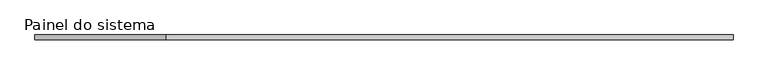
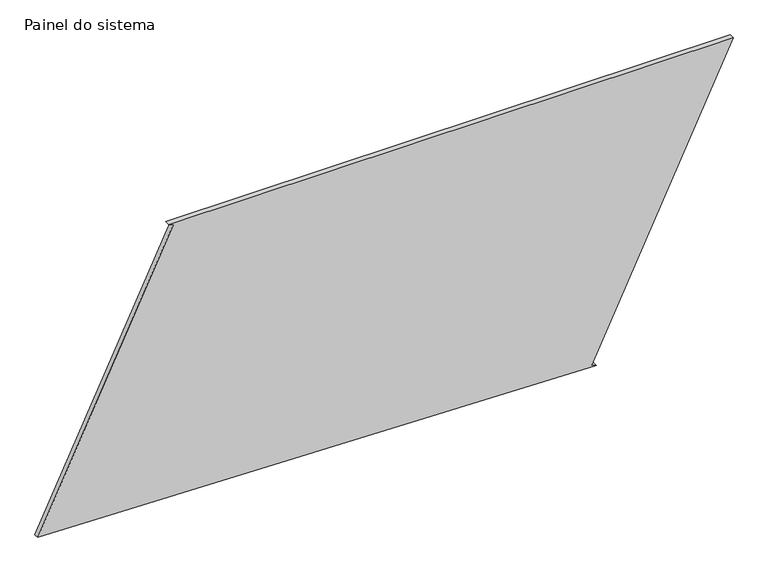
"""IFC4 building model written with IfcOpenShell, lengths in millimetres: plate geometry, Painel do sistema : Envidraçado."""

from ifc_helpers import new_model, si_unit, frame, origin, place, context, project, spatial, polyline, outline, extrude, source, transform, mapped, element, save


def painel_do_sistema_d71562d0(model_context):
    return source(origin(), model_context, "Body", "SweptSolid", [
        extrude(outline(polyline([(0.0, 1053.0263607), (10.7698497, 1030.4651033), (1493.5264309, 1738.2742973), (1493.5264309, -1084.7387177), (1482.7565812, -1062.1774602), (66.4327426, -1738.2742973), (0.0, 1053.0263607)])), frame((0.0, 24.5, 0.0), z_axis=(0.0, 1.0, 0.0), x_axis=(0.0, 0.0, 1.0)), (0.0, 0.0, 1.0), 25.0),
    ])


if __name__ == "__main__":
    model = new_model("IFC4")
    model_context = context("Model", 3, world=origin())
    ifc_project = project(units=[si_unit("LENGTHUNIT", "METRE", prefix="MILLI")], contexts=[model_context])
    site = spatial("IfcSite", under=ifc_project)
    building = spatial("IfcBuilding", under=site)
    placement = place(None, origin())
    painel_do_sistema_shape = painel_do_sistema_d71562d0(model_context)
    element("IfcPlate", 1, ObjectType="Painel do sistema : Envidraçado", at=placement, inside=building, context=model_context, shape_type="MappedRepresentation", body=[
        mapped(painel_do_sistema_shape, transform((0.0, 0.0, 0.0), x_axis=(1.0, 0.0, 0.0), y_axis=(0.0, 1.0, 0.0), z_axis=(0.0, 0.0, 1.0))),
    ])
    save(model, "model.ifc")

# Revit data of these elements
# Type "Painel do sistema : Envidraçado"
#   Construction Type Id = "GSP4R"
#   Analytic Construction = "Vidraça única Pilkington 1/8 pol"
#   Visual Light Transmittance = 0.9
#   Solar Heat Gain Coefficient = 0.86
#   Heat Transfer Coefficient (U) = 6.7069 W/(m²·K)
# Element 1 (IfcPlate, "Painel do sistema : Envidraçado")
#   Materials on its faces: "Vidro"
# Materials
#   "Vidro": class "Vidro", colour RGB 0 128 192, transparency 0.9, Description = "Vidro de sílica", Cost = 0
